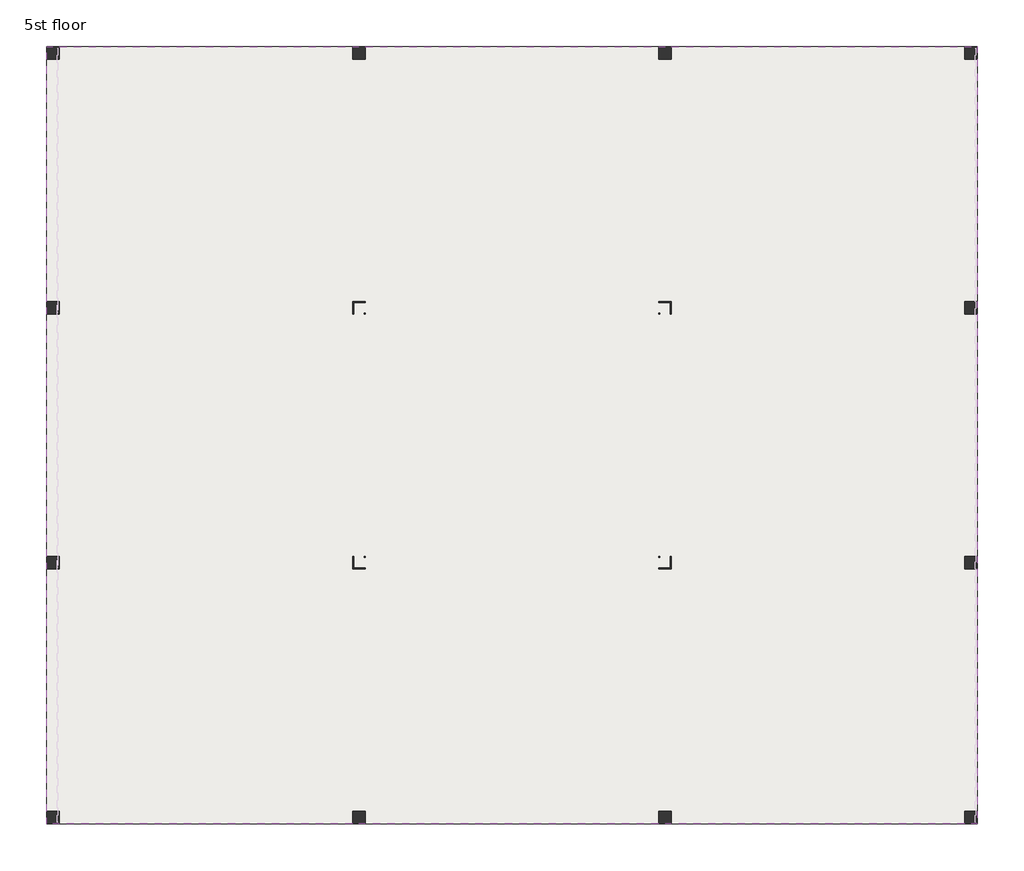
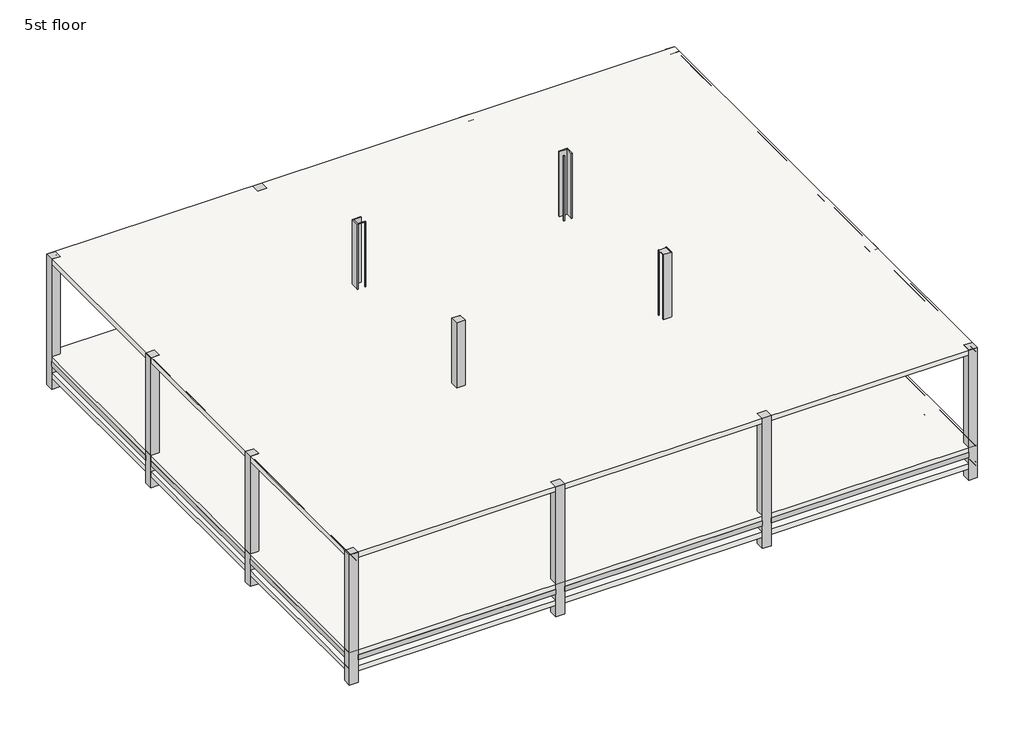
# One storey, part 1 of 2: 24 beams, 16 columns, 3 slabs.
"""IFC4 building model written with IfcOpenShell, lengths in millimetres."""

from ifc_helpers import new_model, si_unit, frame, origin, place, context, project, spatial, polyline, outline, extrude, faceted_brep, element, save

model = new_model("IFC4")

# Units and contexts
model_context = context("Model", 3, world=origin())
ifc_project = project(units=[si_unit("LENGTHUNIT", "METRE", prefix="MILLI")], contexts=[model_context])

# Site, building, storey
site = spatial("IfcSite", under=ifc_project)
building = spatial("IfcBuilding", under=site)
storey = spatial("IfcBuildingStorey", under=building, Name="5st floor", Elevation=19000.0)

# Beams
placement = place(None, origin())
element("IfcBeam", 1, ObjectType="Concrete-Rectangular Beam : 250 x 300mm", at=placement, inside=storey, context=model_context, shape_type="SweptSolid", body=[
    extrude(outline(polyline([(-8833.7181639, -5693.2383613), (-8833.7181639, -5443.2383613), (-3083.7181639, -5443.2383613), (-3083.7181639, -5693.2383613), (-8833.7181639, -5693.2383613)])), frame((0.0, 0.0, 18700.0), z_axis=(0.0, 0.0, 1.0), x_axis=(1.0, 0.0, 0.0)), (0.0, 0.0, 1.0), 150.0),
])
element("IfcBeam", 2, ObjectType="Concrete-Rectangular Beam : 250 x 300mm", at=placement, inside=storey, context=model_context, shape_type="SweptSolid", body=[
    extrude(outline(polyline([(-2833.7181639, -5693.2383613), (-2833.7181639, -5443.2383613), (2916.2818361, -5443.2383613), (2916.2818361, -5693.2383613), (-2833.7181639, -5693.2383613)])), frame((0.0, 0.0, 18700.0), z_axis=(0.0, 0.0, 1.0), x_axis=(1.0, 0.0, 0.0)), (0.0, 0.0, 1.0), 150.0),
])
element("IfcBeam", 3, ObjectType="Concrete-Rectangular Beam : 250 x 300mm", at=placement, inside=storey, context=model_context, shape_type="SweptSolid", body=[
    extrude(outline(polyline([(3166.2818361, -5693.2383613), (3166.2818361, -5443.2383613), (8916.2818361, -5443.2383613), (8916.2818361, -5693.2383613), (3166.2818361, -5693.2383613)])), frame((0.0, 0.0, 18700.0), z_axis=(0.0, 0.0, 1.0), x_axis=(1.0, 0.0, 0.0)), (0.0, 0.0, 1.0), 150.0),
])
element("IfcBeam", 4, ObjectType="Concrete-Rectangular Beam : 250 x 300mm", at=placement, inside=storey, context=model_context, shape_type="SweptSolid", body=[
    extrude(outline(polyline([(-8833.7181639, -10443.2383613), (-9083.7181639, -10443.2383613), (-9083.7181639, -5693.2383613), (-8833.7181639, -5693.2383613), (-8833.7181639, -10443.2383613)])), frame((0.0, 0.0, 18700.0), z_axis=(0.0, 0.0, 1.0), x_axis=(1.0, 0.0, 0.0)), (0.0, 0.0, 1.0), 150.0),
])
element("IfcBeam", 5, ObjectType="Concrete-Rectangular Beam : 250 x 300mm", at=placement, inside=storey, context=model_context, shape_type="SweptSolid", body=[
    extrude(outline(polyline([(-8833.7181639, -15443.2383613), (-9083.7181639, -15443.2383613), (-9083.7181639, -10693.2383613), (-8833.7181639, -10693.2383613), (-8833.7181639, -15443.2383613)])), frame((0.0, 0.0, 18700.0), z_axis=(0.0, 0.0, 1.0), x_axis=(1.0, 0.0, 0.0)), (0.0, 0.0, 1.0), 150.0),
])
element("IfcBeam", 6, ObjectType="Concrete-Rectangular Beam : 250 x 300mm", at=placement, inside=storey, context=model_context, shape_type="SweptSolid", body=[
    extrude(outline(polyline([(-8833.7181639, -20443.2383613), (-9083.7181639, -20443.2383613), (-9083.7181639, -15693.2383613), (-8833.7181639, -15693.2383613), (-8833.7181639, -20443.2383613)])), frame((0.0, 0.0, 18700.0), z_axis=(0.0, 0.0, 1.0), x_axis=(1.0, 0.0, 0.0)), (0.0, 0.0, 1.0), 150.0),
])
element("IfcBeam", 7, ObjectType="Concrete-Rectangular Beam : 250 x 300mm", at=placement, inside=storey, context=model_context, shape_type="SweptSolid", body=[
    extrude(outline(polyline([(-2833.7181639, -10443.2383613), (-3083.7181639, -10443.2383613), (-3083.7181639, -5693.2383613), (-2833.7181639, -5693.2383613), (-2833.7181639, -10443.2383613)])), frame((0.0, 0.0, 18700.0), z_axis=(0.0, 0.0, 1.0), x_axis=(1.0, 0.0, 0.0)), (0.0, 0.0, 1.0), 150.0),
])
element("IfcBeam", 8, ObjectType="Concrete-Rectangular Beam : 250 x 300mm", at=placement, inside=storey, context=model_context, shape_type="SweptSolid", body=[
    extrude(outline(polyline([(-3083.7181639, -15443.2383613), (-3083.7181639, -10693.2383613), (-3058.7181639, -10693.2383613), (-3058.7181639, -15443.2383613), (-3083.7181639, -15443.2383613)])), frame((0.0, 0.0, 18700.0), z_axis=(0.0, 0.0, 1.0), x_axis=(1.0, 0.0, 0.0)), (0.0, 0.0, 1.0), 150.0),
    extrude(outline(polyline([(-2833.7181639, -10693.2383613), (-2833.7181639, -15443.2383613), (-2858.7181639, -15443.2383613), (-2858.7181639, -10693.2383613), (-2833.7181639, -10693.2383613)])), frame((0.0, 0.0, 18700.0), z_axis=(0.0, 0.0, 1.0), x_axis=(1.0, 0.0, 0.0)), (0.0, 0.0, 1.0), 150.0),
])
element("IfcBeam", 9, ObjectType="Concrete-Rectangular Beam : 250 x 300mm", at=placement, inside=storey, context=model_context, shape_type="SweptSolid", body=[
    extrude(outline(polyline([(-2833.7181639, -20443.2383613), (-3083.7181639, -20443.2383613), (-3083.7181639, -15693.2383613), (-2833.7181639, -15693.2383613), (-2833.7181639, -20443.2383613)])), frame((0.0, 0.0, 18700.0), z_axis=(0.0, 0.0, 1.0), x_axis=(1.0, 0.0, 0.0)), (0.0, 0.0, 1.0), 150.0),
])
element("IfcBeam", 10, ObjectType="Concrete-Rectangular Beam : 250 x 300mm", at=placement, inside=storey, context=model_context, shape_type="SweptSolid", body=[
    extrude(outline(polyline([(3166.2818361, -10443.2383613), (2916.2818361, -10443.2383613), (2916.2818361, -5693.2383613), (3166.2818361, -5693.2383613), (3166.2818361, -10443.2383613)])), frame((0.0, 0.0, 18700.0), z_axis=(0.0, 0.0, 1.0), x_axis=(1.0, 0.0, 0.0)), (0.0, 0.0, 1.0), 150.0),
])
element("IfcBeam", 11, ObjectType="Concrete-Rectangular Beam : 250 x 300mm", at=placement, inside=storey, context=model_context, shape_type="SweptSolid", body=[
    extrude(outline(polyline([(2916.2818361, -15443.2383613), (2916.2818361, -10693.2383613), (2941.2818361, -10693.2383613), (2941.2818361, -15443.2383613), (2916.2818361, -15443.2383613)])), frame((0.0, 0.0, 18700.0), z_axis=(0.0, 0.0, 1.0), x_axis=(1.0, 0.0, 0.0)), (0.0, 0.0, 1.0), 150.0),
    extrude(outline(polyline([(3166.2818361, -10693.2383613), (3166.2818361, -15443.2383613), (3141.2818361, -15443.2383613), (3141.2818361, -10693.2383613), (3166.2818361, -10693.2383613)])), frame((0.0, 0.0, 18700.0), z_axis=(0.0, 0.0, 1.0), x_axis=(1.0, 0.0, 0.0)), (0.0, 0.0, 1.0), 150.0),
])
element("IfcBeam", 12, ObjectType="Concrete-Rectangular Beam : 250 x 300mm", at=placement, inside=storey, context=model_context, shape_type="SweptSolid", body=[
    extrude(outline(polyline([(3166.2818361, -20443.2383613), (2916.2818361, -20443.2383613), (2916.2818361, -15693.2383613), (3166.2818361, -15693.2383613), (3166.2818361, -20443.2383613)])), frame((0.0, 0.0, 18700.0), z_axis=(0.0, 0.0, 1.0), x_axis=(1.0, 0.0, 0.0)), (0.0, 0.0, 1.0), 150.0),
])
element("IfcBeam", 13, ObjectType="Concrete-Rectangular Beam : 250 x 300mm", at=placement, inside=storey, context=model_context, shape_type="SweptSolid", body=[
    extrude(outline(polyline([(9166.2818361, -10443.2383613), (8916.2818361, -10443.2383613), (8916.2818361, -5693.2383613), (9166.2818361, -5693.2383613), (9166.2818361, -10443.2383613)])), frame((0.0, 0.0, 18700.0), z_axis=(0.0, 0.0, 1.0), x_axis=(1.0, 0.0, 0.0)), (0.0, 0.0, 1.0), 150.0),
])
element("IfcBeam", 14, ObjectType="Concrete-Rectangular Beam : 250 x 300mm", at=placement, inside=storey, context=model_context, shape_type="SweptSolid", body=[
    extrude(outline(polyline([(9166.2818361, -15443.2383613), (8916.2818361, -15443.2383613), (8916.2818361, -10693.2383613), (9166.2818361, -10693.2383613), (9166.2818361, -15443.2383613)])), frame((0.0, 0.0, 18700.0), z_axis=(0.0, 0.0, 1.0), x_axis=(1.0, 0.0, 0.0)), (0.0, 0.0, 1.0), 150.0),
])
element("IfcBeam", 15, ObjectType="Concrete-Rectangular Beam : 250 x 300mm", at=placement, inside=storey, context=model_context, shape_type="SweptSolid", body=[
    extrude(outline(polyline([(9166.2818361, -20443.2383613), (8916.2818361, -20443.2383613), (8916.2818361, -15693.2383613), (9166.2818361, -15693.2383613), (9166.2818361, -20443.2383613)])), frame((0.0, 0.0, 18700.0), z_axis=(0.0, 0.0, 1.0), x_axis=(1.0, 0.0, 0.0)), (0.0, 0.0, 1.0), 150.0),
])
element("IfcBeam", 16, ObjectType="Concrete-Rectangular Beam : 250 x 300mm", at=placement, inside=storey, context=model_context, shape_type="SweptSolid", body=[
    extrude(outline(polyline([(-8833.7181639, -20693.2383613), (-8833.7181639, -20443.2383613), (-3083.7181639, -20443.2383613), (-3083.7181639, -20693.2383613), (-8833.7181639, -20693.2383613)])), frame((0.0, 0.0, 18700.0), z_axis=(0.0, 0.0, 1.0), x_axis=(1.0, 0.0, 0.0)), (0.0, 0.0, 1.0), 150.0),
])
element("IfcBeam", 17, ObjectType="Concrete-Rectangular Beam : 250 x 300mm", at=placement, inside=storey, context=model_context, shape_type="SweptSolid", body=[
    extrude(outline(polyline([(-2833.7181639, -20693.2383613), (-2833.7181639, -20443.2383613), (2916.2818361, -20443.2383613), (2916.2818361, -20693.2383613), (-2833.7181639, -20693.2383613)])), frame((0.0, 0.0, 18700.0), z_axis=(0.0, 0.0, 1.0), x_axis=(1.0, 0.0, 0.0)), (0.0, 0.0, 1.0), 150.0),
])
element("IfcBeam", 18, ObjectType="Concrete-Rectangular Beam : 250 x 300mm", at=placement, inside=storey, context=model_context, shape_type="SweptSolid", body=[
    extrude(outline(polyline([(3166.2818361, -20693.2383613), (3166.2818361, -20443.2383613), (8916.2818361, -20443.2383613), (8916.2818361, -20693.2383613), (3166.2818361, -20693.2383613)])), frame((0.0, 0.0, 18700.0), z_axis=(0.0, 0.0, 1.0), x_axis=(1.0, 0.0, 0.0)), (0.0, 0.0, 1.0), 150.0),
])
element("IfcBeam", 19, ObjectType="Concrete-Rectangular Beam : 250 x 300mm", at=placement, inside=storey, context=model_context, shape_type="SweptSolid", body=[
    extrude(outline(polyline([(-8833.7181639, -15693.2383613), (-8833.7181639, -15443.2383613), (-3083.7181639, -15443.2383613), (-3083.7181639, -15693.2383613), (-8833.7181639, -15693.2383613)])), frame((0.0, 0.0, 18700.0), z_axis=(0.0, 0.0, 1.0), x_axis=(1.0, 0.0, 0.0)), (0.0, 0.0, 1.0), 150.0),
])
element("IfcBeam", 20, ObjectType="Concrete-Rectangular Beam : 250 x 300mm", at=placement, inside=storey, context=model_context, shape_type="SweptSolid", body=[
    extrude(outline(polyline([(2916.2818361, -15693.2383613), (-2833.7181639, -15693.2383613), (-2833.7181639, -15668.2383613), (2916.2818361, -15668.2383613), (2916.2818361, -15693.2383613)])), frame((0.0, 0.0, 18700.0), z_axis=(0.0, 0.0, 1.0), x_axis=(1.0, 0.0, 0.0)), (0.0, 0.0, 1.0), 150.0),
    extrude(outline(polyline([(-2833.7181639, -15443.2383613), (2916.2818361, -15443.2383613), (2916.2818361, -15468.2383613), (-2833.7181639, -15468.2383613), (-2833.7181639, -15443.2383613)])), frame((0.0, 0.0, 18700.0), z_axis=(0.0, 0.0, 1.0), x_axis=(1.0, 0.0, 0.0)), (0.0, 0.0, 1.0), 150.0),
])
element("IfcBeam", 21, ObjectType="Concrete-Rectangular Beam : 250 x 300mm", at=placement, inside=storey, context=model_context, shape_type="SweptSolid", body=[
    extrude(outline(polyline([(3166.2818361, -15693.2383613), (3166.2818361, -15443.2383613), (8916.2818361, -15443.2383613), (8916.2818361, -15693.2383613), (3166.2818361, -15693.2383613)])), frame((0.0, 0.0, 18700.0), z_axis=(0.0, 0.0, 1.0), x_axis=(1.0, 0.0, 0.0)), (0.0, 0.0, 1.0), 150.0),
])
element("IfcBeam", 22, ObjectType="Concrete-Rectangular Beam : 250 x 300mm", at=placement, inside=storey, context=model_context, shape_type="SweptSolid", body=[
    extrude(outline(polyline([(-8833.7181639, -10693.2383613), (-8833.7181639, -10443.2383613), (-3083.7181639, -10443.2383613), (-3083.7181639, -10693.2383613), (-8833.7181639, -10693.2383613)])), frame((0.0, 0.0, 18700.0), z_axis=(0.0, 0.0, 1.0), x_axis=(1.0, 0.0, 0.0)), (0.0, 0.0, 1.0), 150.0),
])
element("IfcBeam", 23, ObjectType="Concrete-Rectangular Beam : 250 x 300mm", at=placement, inside=storey, context=model_context, shape_type="SweptSolid", body=[
    extrude(outline(polyline([(2916.2818361, -10693.2383613), (-2833.7181639, -10693.2383613), (-2833.7181639, -10668.2383613), (2916.2818361, -10668.2383613), (2916.2818361, -10693.2383613)])), frame((0.0, 0.0, 18700.0), z_axis=(0.0, 0.0, 1.0), x_axis=(1.0, 0.0, 0.0)), (0.0, 0.0, 1.0), 150.0),
    extrude(outline(polyline([(-2833.7181639, -10443.2383613), (2916.2818361, -10443.2383613), (2916.2818361, -10468.2383613), (-2833.7181639, -10468.2383613), (-2833.7181639, -10443.2383613)])), frame((0.0, 0.0, 18700.0), z_axis=(0.0, 0.0, 1.0), x_axis=(1.0, 0.0, 0.0)), (0.0, 0.0, 1.0), 150.0),
])
element("IfcBeam", 24, ObjectType="Concrete-Rectangular Beam : 250 x 300mm", at=placement, inside=storey, context=model_context, shape_type="SweptSolid", body=[
    extrude(outline(polyline([(3166.2818361, -10693.2383613), (3166.2818361, -10443.2383613), (8916.2818361, -10443.2383613), (8916.2818361, -10693.2383613), (3166.2818361, -10693.2383613)])), frame((0.0, 0.0, 18700.0), z_axis=(0.0, 0.0, 1.0), x_axis=(1.0, 0.0, 0.0)), (0.0, 0.0, 1.0), 150.0),
])

# Columns
element("IfcColumn", 25, ObjectType="Concrete-Rectangular-Column : 250x250 mm", at=placement, inside=storey, context=model_context, shape_type="Brep", body=[
    faceted_brep([(-8833.7181639, -20443.2383613, 22000.0), (-9083.7181639, -20443.2383613, 22000.0), (-9083.7181639, -20693.2383613, 22000.0), (-8833.7181639, -20693.2383613, 22000.0), (-8833.7181639, -20443.2383613, 18000.0), (-8833.7181639, -20693.2383613, 18000.0), (-9083.7181639, -20693.2383613, 18000.0), (-9083.7181639, -20443.2383613, 18000.0), (-8833.7181639, -20443.2383613, 18350.0), (-8833.7181639, -20443.2383613, 18200.0), (-9083.7181639, -20443.2383613, 18200.0), (-9083.7181639, -20443.2383613, 18350.0), (-8833.7181639, -20693.2383613, 18200.0), (-8833.7181639, -20693.2383613, 18350.0)], [[[0, 1, 2, 3]], [[4, 5, 6, 7]], [[1, 0, 8, 9, 4, 7, 10, 11]], [[2, 1, 11, 10, 7, 6]], [[3, 2, 6, 5, 12, 13]], [[0, 3, 13, 12, 5, 4, 9, 8]]]),
])
element("IfcColumn", 26, ObjectType="Concrete-Rectangular-Column : 250x250 mm", at=placement, inside=storey, context=model_context, shape_type="Brep", body=[
    faceted_brep([(-8833.7181639, -15443.2383613, 22000.0), (-9083.7181639, -15443.2383613, 22000.0), (-9083.7181639, -15693.2383613, 22000.0), (-8833.7181639, -15693.2383613, 22000.0), (-8833.7181639, -15443.2383613, 18000.0), (-8833.7181639, -15693.2383613, 18000.0), (-9083.7181639, -15693.2383613, 18000.0), (-9083.7181639, -15443.2383613, 18000.0), (-8833.7181639, -15443.2383613, 18350.0), (-8833.7181639, -15443.2383613, 18200.0), (-9083.7181639, -15443.2383613, 18200.0), (-9083.7181639, -15443.2383613, 18350.0), (-9083.7181639, -15693.2383613, 18200.0), (-9083.7181639, -15693.2383613, 18350.0), (-8833.7181639, -15693.2383613, 18200.0), (-8833.7181639, -15693.2383613, 18350.0)], [[[0, 1, 2, 3]], [[4, 5, 6, 7]], [[1, 0, 8, 9, 4, 7, 10, 11]], [[2, 1, 11, 10, 7, 6, 12, 13]], [[3, 2, 13, 12, 6, 5, 14, 15]], [[0, 3, 15, 14, 5, 4, 9, 8]]]),
])
element("IfcColumn", 27, ObjectType="Concrete-Rectangular-Column : 250x250 mm", at=placement, inside=storey, context=model_context, shape_type="Brep", body=[
    faceted_brep([(-8833.7181639, -10443.2383613, 22000.0), (-9083.7181639, -10443.2383613, 22000.0), (-9083.7181639, -10693.2383613, 22000.0), (-8833.7181639, -10693.2383613, 22000.0), (-8833.7181639, -10443.2383613, 18000.0), (-8833.7181639, -10693.2383613, 18000.0), (-9083.7181639, -10693.2383613, 18000.0), (-9083.7181639, -10443.2383613, 18000.0), (-8833.7181639, -10443.2383613, 18350.0), (-8833.7181639, -10443.2383613, 18200.0), (-9083.7181639, -10443.2383613, 18200.0), (-9083.7181639, -10443.2383613, 18350.0), (-9083.7181639, -10693.2383613, 18200.0), (-9083.7181639, -10693.2383613, 18350.0), (-8833.7181639, -10693.2383613, 18200.0), (-8833.7181639, -10693.2383613, 18350.0)], [[[0, 1, 2, 3]], [[4, 5, 6, 7]], [[1, 0, 8, 9, 4, 7, 10, 11]], [[2, 1, 11, 10, 7, 6, 12, 13]], [[3, 2, 13, 12, 6, 5, 14, 15]], [[0, 3, 15, 14, 5, 4, 9, 8]]]),
])
element("IfcColumn", 28, ObjectType="Concrete-Rectangular-Column : 250x250 mm", at=placement, inside=storey, context=model_context, shape_type="Brep", body=[
    faceted_brep([(-8833.7181639, -5443.2383613, 22000.0), (-9083.7181639, -5443.2383613, 22000.0), (-9083.7181639, -5693.2383613, 22000.0), (-8833.7181639, -5693.2383613, 22000.0), (-8833.7181639, -5443.2383613, 18000.0), (-8833.7181639, -5693.2383613, 18000.0), (-9083.7181639, -5693.2383613, 18000.0), (-9083.7181639, -5443.2383613, 18000.0), (-8833.7181639, -5443.2383613, 18350.0), (-8833.7181639, -5443.2383613, 18200.0), (-9083.7181639, -5693.2383613, 18200.0), (-9083.7181639, -5693.2383613, 18350.0), (-8833.7181639, -5693.2383613, 18200.0), (-8833.7181639, -5693.2383613, 18350.0)], [[[0, 1, 2, 3]], [[4, 5, 6, 7]], [[1, 0, 8, 9, 4, 7]], [[2, 1, 7, 6, 10, 11]], [[3, 2, 11, 10, 6, 5, 12, 13]], [[0, 3, 13, 12, 5, 4, 9, 8]]]),
])
element("IfcColumn", 29, ObjectType="Concrete-Rectangular-Column : 250x250 mm", at=placement, inside=storey, context=model_context, shape_type="Brep", body=[
    faceted_brep([(-2833.7181639, -20443.2383613, 22000.0), (-3083.7181639, -20443.2383613, 22000.0), (-3083.7181639, -20693.2383613, 22000.0), (-2833.7181639, -20693.2383613, 22000.0), (-2833.7181639, -20443.2383613, 18000.0), (-2833.7181639, -20693.2383613, 18000.0), (-3083.7181639, -20693.2383613, 18000.0), (-3083.7181639, -20443.2383613, 18000.0), (-2833.7181639, -20443.2383613, 18350.0), (-2833.7181639, -20443.2383613, 18200.0), (-3083.7181639, -20443.2383613, 18200.0), (-3083.7181639, -20443.2383613, 18350.0), (-3083.7181639, -20693.2383613, 18200.0), (-3083.7181639, -20693.2383613, 18350.0), (-2833.7181639, -20693.2383613, 18200.0), (-2833.7181639, -20693.2383613, 18350.0)], [[[0, 1, 2, 3]], [[4, 5, 6, 7]], [[1, 0, 8, 9, 4, 7, 10, 11]], [[2, 1, 11, 10, 7, 6, 12, 13]], [[3, 2, 13, 12, 6, 5, 14, 15]], [[0, 3, 15, 14, 5, 4, 9, 8]]]),
])
element("IfcColumn", 30, ObjectType="Concrete-Rectangular-Column : 250x250 mm", at=placement, inside=storey, context=model_context, shape_type="Brep", body=[
    faceted_brep([(-2833.7181639, -15443.2383613, 24000.0), (-3083.7181639, -15443.2383613, 24000.0), (-3083.7181639, -15693.2383613, 24000.0), (-2833.7181639, -15693.2383613, 24000.0), (-2833.7181639, -15443.2383613, 18000.0), (-2833.7181639, -15468.2383613, 18000.0), (-2858.7181639, -15468.2383613, 18000.0), (-2858.7181639, -15443.2383613, 18000.0), (-2833.7181639, -15443.2383613, 18350.0), (-2833.7181639, -15443.2383613, 18200.0), (-2858.7181639, -15443.2383613, 18200.0), (-2858.7181639, -15443.2383613, 18350.0), (-2858.7181639, -15443.2383613, 23998.7852478), (-3058.7181639, -15443.2383613, 23998.7852478), (-3058.7181639, -15443.2383613, 18350.0), (-3058.7181639, -15443.2383613, 18200.0), (-3058.7181639, -15443.2383613, 18000.0), (-3083.7181639, -15443.2383613, 18000.0), (-3083.7181639, -15443.2383613, 18200.0), (-3083.7181639, -15443.2383613, 18350.0), (-3083.7181639, -15693.2383613, 18000.0), (-3083.7181639, -15693.2383613, 18200.0), (-3083.7181639, -15693.2383613, 18350.0), (-2833.7181639, -15693.2383613, 18000.0), (-2833.7181639, -15693.2383613, 18200.0), (-2833.7181639, -15693.2383613, 18350.0), (-2833.7181639, -15668.2383613, 18000.0), (-2833.7181639, -15668.2383613, 18200.0), (-2833.7181639, -15668.2383613, 18350.0), (-2833.7181639, -15668.2383613, 23998.7852478), (-2833.7181639, -15468.2383613, 23998.7852478), (-2833.7181639, -15468.2383613, 18350.0), (-2833.7181639, -15468.2383613, 18200.0), (-2858.7181639, -15468.2383613, 23998.7852478), (-3058.7181639, -15668.2383613, 18000.0), (-3058.7181639, -15668.2383613, 23998.7852478), (-3058.7181639, -15468.2383613, 23998.7852478)], [[[0, 1, 2, 3]], [[4, 5, 6, 7]], [[1, 0, 8, 9, 4, 7, 10, 11, 12, 13, 14, 15, 16, 17, 18, 19]], [[2, 1, 19, 18, 17, 20, 21, 22]], [[3, 2, 22, 21, 20, 23, 24, 25]], [[0, 3, 25, 24, 23, 26, 27, 28, 29, 30, 31, 32, 5, 4, 9, 8]], [[5, 32, 31, 30, 33, 6]], [[34, 35, 29, 28, 27, 26]], [[35, 34, 16, 15, 14, 13, 36]], [[33, 12, 11, 10, 7, 6]], [[23, 20, 17, 16, 34, 26]], [[35, 36, 13, 12, 33, 30, 29]]]),
])
element("IfcColumn", 31, ObjectType="Concrete-Rectangular-Column : 250x250 mm", at=placement, inside=storey, context=model_context, shape_type="Brep", body=[
    faceted_brep([(-2833.7181639, -10443.2383613, 24000.0), (-3083.7181639, -10443.2383613, 24000.0), (-3083.7181639, -10693.2383613, 24000.0), (-2833.7181639, -10693.2383613, 24000.0), (-2833.7181639, -10668.2383613, 24000.0), (-3058.7181639, -10668.2383613, 24000.0), (-3058.7181639, -10468.2383613, 24000.0), (-2833.7181639, -10468.2383613, 24000.0), (-3083.7181639, -10693.2383613, 18000.0), (-3083.7181639, -10443.2383613, 18000.0), (-2833.7181639, -10443.2383613, 18000.0), (-2833.7181639, -10468.2383613, 18000.0), (-3058.7181639, -10468.2383613, 18000.0), (-3058.7181639, -10693.2383613, 18000.0), (-2833.7181639, -10443.2383613, 18350.0), (-2833.7181639, -10443.2383613, 18200.0), (-3083.7181639, -10443.2383613, 18200.0), (-3083.7181639, -10443.2383613, 18350.0), (-3083.7181639, -10693.2383613, 18200.0), (-3083.7181639, -10693.2383613, 18350.0), (-3058.7181639, -10693.2383613, 18200.0), (-3058.7181639, -10693.2383613, 18350.0), (-3058.7181639, -10693.2383613, 23998.7852478), (-2858.7181639, -10693.2383613, 23998.7852478), (-2858.7181639, -10693.2383613, 18350.0), (-2858.7181639, -10693.2383613, 18200.0), (-2858.7181639, -10693.2383613, 18000.0), (-2833.7181639, -10693.2383613, 18000.0), (-2833.7181639, -10693.2383613, 18200.0), (-2833.7181639, -10693.2383613, 18350.0), (-2833.7181639, -10468.2383613, 18350.0), (-2833.7181639, -10468.2383613, 18200.0), (-2833.7181639, -10668.2383613, 18350.0), (-2833.7181639, -10668.2383613, 18200.0), (-2833.7181639, -10668.2383613, 18000.0), (-2858.7181639, -10668.2383613, 18000.0), (-2858.7181639, -10668.2383613, 23998.7852478), (-3058.7181639, -10668.2383613, 23998.7852478)], [[[0, 1, 2, 3, 4, 5, 6, 7]], [[8, 9, 10, 11, 12, 13]], [[1, 0, 14, 15, 10, 9, 16, 17]], [[2, 1, 17, 16, 9, 8, 18, 19]], [[3, 2, 19, 18, 8, 13, 20, 21, 22, 23, 24, 25, 26, 27, 28, 29]], [[10, 15, 14, 0, 7, 30, 31, 11]], [[4, 32, 33, 34, 35, 36, 37, 5]], [[12, 11, 31, 30, 7, 6]], [[12, 6, 5, 37, 22, 21, 20, 13]], [[23, 36, 35, 26, 25, 24]], [[34, 27, 26, 35]], [[3, 29, 28, 27, 34, 33, 32, 4]], [[22, 37, 36, 23]]]),
])
element("IfcColumn", 32, ObjectType="Concrete-Rectangular-Column : 250x250 mm", at=placement, inside=storey, context=model_context, shape_type="Brep", body=[
    faceted_brep([(-2833.7181639, -5443.2383613, 22000.0), (-3083.7181639, -5443.2383613, 22000.0), (-3083.7181639, -5693.2383613, 22000.0), (-2833.7181639, -5693.2383613, 22000.0), (-2833.7181639, -5443.2383613, 18000.0), (-2833.7181639, -5693.2383613, 18000.0), (-3083.7181639, -5693.2383613, 18000.0), (-3083.7181639, -5443.2383613, 18000.0), (-2833.7181639, -5443.2383613, 18350.0), (-2833.7181639, -5443.2383613, 18200.0), (-3083.7181639, -5443.2383613, 18200.0), (-3083.7181639, -5443.2383613, 18350.0), (-3083.7181639, -5693.2383613, 18200.0), (-3083.7181639, -5693.2383613, 18350.0), (-2833.7181639, -5693.2383613, 18200.0), (-2833.7181639, -5693.2383613, 18350.0)], [[[0, 1, 2, 3]], [[4, 5, 6, 7]], [[1, 0, 8, 9, 4, 7, 10, 11]], [[2, 1, 11, 10, 7, 6, 12, 13]], [[3, 2, 13, 12, 6, 5, 14, 15]], [[0, 3, 15, 14, 5, 4, 9, 8]]]),
])
element("IfcColumn", 33, ObjectType="Concrete-Rectangular-Column : 250x250 mm", at=placement, inside=storey, context=model_context, shape_type="Brep", body=[
    faceted_brep([(3166.2818361, -20443.2383613, 22000.0), (2916.2818361, -20443.2383613, 22000.0), (2916.2818361, -20693.2383613, 22000.0), (3166.2818361, -20693.2383613, 22000.0), (3166.2818361, -20443.2383613, 18000.0), (3166.2818361, -20693.2383613, 18000.0), (2916.2818361, -20693.2383613, 18000.0), (2916.2818361, -20443.2383613, 18000.0), (3166.2818361, -20443.2383613, 18350.0), (3166.2818361, -20443.2383613, 18200.0), (2916.2818361, -20443.2383613, 18200.0), (2916.2818361, -20443.2383613, 18350.0), (2916.2818361, -20693.2383613, 18200.0), (2916.2818361, -20693.2383613, 18350.0), (3166.2818361, -20693.2383613, 18200.0), (3166.2818361, -20693.2383613, 18350.0)], [[[0, 1, 2, 3]], [[4, 5, 6, 7]], [[1, 0, 8, 9, 4, 7, 10, 11]], [[2, 1, 11, 10, 7, 6, 12, 13]], [[3, 2, 13, 12, 6, 5, 14, 15]], [[0, 3, 15, 14, 5, 4, 9, 8]]]),
])
element("IfcColumn", 34, ObjectType="Concrete-Rectangular-Column : 250x250 mm", at=placement, inside=storey, context=model_context, shape_type="Brep", body=[
    faceted_brep([(2916.2818361, -15443.2383613, 24000.0), (2916.2818361, -15693.2383613, 24000.0), (3166.2818361, -15693.2383613, 24000.0), (3166.2818361, -15443.2383613, 24000.0), (3141.2818361, -15443.2383613, 24000.0), (3141.2818361, -15468.2383613, 24000.0), (2941.2818361, -15468.2383613, 24000.0), (2941.2818361, -15443.2383613, 24000.0), (2916.2818361, -15468.2383613, 18000.0), (2916.2818361, -15443.2383613, 18000.0), (2941.2818361, -15443.2383613, 18000.0), (2941.2818361, -15468.2383613, 18000.0), (3166.2818361, -15443.2383613, 18350.0), (3166.2818361, -15443.2383613, 18200.0), (3166.2818361, -15443.2383613, 18000.0), (3141.2818361, -15443.2383613, 18000.0), (3141.2818361, -15443.2383613, 18200.0), (3141.2818361, -15443.2383613, 18350.0), (2916.2818361, -15443.2383613, 18350.0), (2916.2818361, -15443.2383613, 18200.0), (2916.2818361, -15468.2383613, 18200.0), (2916.2818361, -15468.2383613, 18350.0), (2916.2818361, -15468.2383613, 23998.7852478), (2916.2818361, -15668.2383613, 23998.7852478), (2916.2818361, -15668.2383613, 18350.0), (2916.2818361, -15668.2383613, 18200.0), (2916.2818361, -15668.2383613, 18000.0), (2916.2818361, -15693.2383613, 18000.0), (2916.2818361, -15693.2383613, 18200.0), (2916.2818361, -15693.2383613, 18350.0), (3166.2818361, -15693.2383613, 18000.0), (3166.2818361, -15693.2383613, 18200.0), (3166.2818361, -15693.2383613, 18350.0), (2941.2818361, -15468.2383613, 23998.7852478), (3141.2818361, -15668.2383613, 23998.7852478), (3141.2818361, -15668.2383613, 18000.0), (3141.2818361, -15468.2383613, 23998.7852478), (2941.2818361, -15443.2383613, 18200.0), (2941.2818361, -15443.2383613, 18350.0)], [[[0, 1, 2, 3, 4, 5, 6, 7]], [[8, 9, 10, 11]], [[3, 12, 13, 14, 15, 16, 17, 4]], [[1, 0, 18, 19, 9, 8, 20, 21, 22, 23, 24, 25, 26, 27, 28, 29]], [[2, 1, 29, 28, 27, 30, 31, 32]], [[3, 2, 32, 31, 30, 14, 13, 12]], [[22, 21, 20, 8, 11, 33]], [[34, 35, 26, 25, 24, 23]], [[34, 36, 5, 4, 17, 16, 15, 35]], [[6, 33, 11, 10, 37, 38, 7]], [[5, 36, 33, 6]], [[14, 30, 27, 26, 35, 15]], [[9, 19, 18, 0, 7, 38, 37, 10]], [[36, 34, 23, 22, 33]]]),
])
element("IfcColumn", 35, ObjectType="Concrete-Rectangular-Column : 250x250 mm", at=placement, inside=storey, context=model_context, shape_type="Brep", body=[
    faceted_brep([(3166.2818361, -10443.2383613, 24000.0), (2916.2818361, -10443.2383613, 24000.0), (2916.2818361, -10468.2383613, 24000.0), (3141.2818361, -10468.2383613, 24000.0), (3141.2818361, -10693.2383613, 24000.0), (3166.2818361, -10693.2383613, 24000.0), (3166.2818361, -10443.2383613, 18350.0), (3166.2818361, -10443.2383613, 18200.0), (3166.2818361, -10443.2383613, 18000.0), (2916.2818361, -10443.2383613, 18000.0), (2916.2818361, -10443.2383613, 18200.0), (2916.2818361, -10443.2383613, 18350.0), (2916.2818361, -10468.2383613, 18000.0), (2916.2818361, -10468.2383613, 18200.0), (2916.2818361, -10468.2383613, 18350.0), (3166.2818361, -10693.2383613, 18350.0), (3166.2818361, -10693.2383613, 18200.0), (3166.2818361, -10693.2383613, 18000.0), (3141.2818361, -10468.2383613, 18000.0), (3141.2818361, -10693.2383613, 18000.0), (3141.2818361, -10693.2383613, 18200.0), (3141.2818361, -10693.2383613, 18350.0)], [[[0, 1, 2, 3, 4, 5]], [[1, 0, 6, 7, 8, 9, 10, 11]], [[1, 11, 10, 9, 12, 13, 14, 2]], [[0, 5, 15, 16, 17, 8, 7, 6]], [[12, 18, 3, 2, 14, 13]], [[19, 20, 21, 4, 3, 18]], [[8, 17, 19, 18, 12, 9]], [[17, 16, 15, 5, 4, 21, 20, 19]]]),
    faceted_brep([(2916.2818361, -10693.2383613, 18000.0), (2916.2818361, -10668.2383613, 18000.0), (2941.2818361, -10668.2383613, 18000.0), (2941.2818361, -10693.2383613, 18000.0), (2916.2818361, -10693.2383613, 24000.0), (2916.2818361, -10693.2383613, 18350.0), (2916.2818361, -10693.2383613, 18200.0), (2941.2818361, -10693.2383613, 18200.0), (2941.2818361, -10693.2383613, 18350.0), (2941.2818361, -10693.2383613, 24000.0), (2916.2818361, -10668.2383613, 18200.0), (2916.2818361, -10668.2383613, 18350.0), (2916.2818361, -10668.2383613, 24000.0), (2941.2818361, -10668.2383613, 24000.0)], [[[0, 1, 2, 3]], [[4, 5, 6, 0, 3, 7, 8, 9]], [[1, 10, 11, 12, 13, 2]], [[13, 9, 8, 7, 3, 2]], [[0, 6, 5, 4, 12, 11, 10, 1]], [[12, 4, 9, 13]]]),
])
element("IfcColumn", 36, ObjectType="Concrete-Rectangular-Column : 250x250 mm", at=placement, inside=storey, context=model_context, shape_type="Brep", body=[
    faceted_brep([(3166.2818361, -5443.2383613, 22000.0), (2916.2818361, -5443.2383613, 22000.0), (2916.2818361, -5693.2383613, 22000.0), (3166.2818361, -5693.2383613, 22000.0), (3166.2818361, -5443.2383613, 18000.0), (3166.2818361, -5693.2383613, 18000.0), (2916.2818361, -5693.2383613, 18000.0), (2916.2818361, -5443.2383613, 18000.0), (3166.2818361, -5443.2383613, 18350.0), (3166.2818361, -5443.2383613, 18200.0), (2916.2818361, -5443.2383613, 18200.0), (2916.2818361, -5443.2383613, 18350.0), (2916.2818361, -5693.2383613, 18200.0), (2916.2818361, -5693.2383613, 18350.0), (3166.2818361, -5693.2383613, 18200.0), (3166.2818361, -5693.2383613, 18350.0)], [[[0, 1, 2, 3]], [[4, 5, 6, 7]], [[1, 0, 8, 9, 4, 7, 10, 11]], [[2, 1, 11, 10, 7, 6, 12, 13]], [[3, 2, 13, 12, 6, 5, 14, 15]], [[0, 3, 15, 14, 5, 4, 9, 8]]]),
])
element("IfcColumn", 37, ObjectType="Concrete-Rectangular-Column : 250x250 mm", at=placement, inside=storey, context=model_context, shape_type="Brep", body=[
    faceted_brep([(9166.2818361, -20443.2383613, 22000.0), (8916.2818361, -20443.2383613, 22000.0), (8916.2818361, -20693.2383613, 22000.0), (9166.2818361, -20693.2383613, 22000.0), (9166.2818361, -20443.2383613, 18000.0), (9166.2818361, -20693.2383613, 18000.0), (8916.2818361, -20693.2383613, 18000.0), (8916.2818361, -20443.2383613, 18000.0), (9166.2818361, -20443.2383613, 18350.0), (9166.2818361, -20443.2383613, 18200.0), (8916.2818361, -20443.2383613, 18200.0), (8916.2818361, -20443.2383613, 18350.0), (8916.2818361, -20693.2383613, 18200.0), (8916.2818361, -20693.2383613, 18350.0)], [[[0, 1, 2, 3]], [[4, 5, 6, 7]], [[1, 0, 8, 9, 4, 7, 10, 11]], [[2, 1, 11, 10, 7, 6, 12, 13]], [[3, 2, 13, 12, 6, 5]], [[0, 3, 5, 4, 9, 8]]]),
])
element("IfcColumn", 38, ObjectType="Concrete-Rectangular-Column : 250x250 mm", at=placement, inside=storey, context=model_context, shape_type="Brep", body=[
    faceted_brep([(9166.2818361, -15443.2383613, 22000.0), (8916.2818361, -15443.2383613, 22000.0), (8916.2818361, -15693.2383613, 22000.0), (9166.2818361, -15693.2383613, 22000.0), (9166.2818361, -15443.2383613, 18000.0), (9166.2818361, -15693.2383613, 18000.0), (8916.2818361, -15693.2383613, 18000.0), (8916.2818361, -15443.2383613, 18000.0), (9166.2818361, -15443.2383613, 18350.0), (9166.2818361, -15443.2383613, 18200.0), (8916.2818361, -15443.2383613, 18200.0), (8916.2818361, -15443.2383613, 18350.0), (8916.2818361, -15693.2383613, 18200.0), (8916.2818361, -15693.2383613, 18350.0), (9166.2818361, -15693.2383613, 18200.0), (9166.2818361, -15693.2383613, 18350.0)], [[[0, 1, 2, 3]], [[4, 5, 6, 7]], [[1, 0, 8, 9, 4, 7, 10, 11]], [[2, 1, 11, 10, 7, 6, 12, 13]], [[3, 2, 13, 12, 6, 5, 14, 15]], [[0, 3, 15, 14, 5, 4, 9, 8]]]),
])
element("IfcColumn", 39, ObjectType="Concrete-Rectangular-Column : 250x250 mm", at=placement, inside=storey, context=model_context, shape_type="Brep", body=[
    faceted_brep([(9166.2818361, -10443.2383613, 22000.0), (8916.2818361, -10443.2383613, 22000.0), (8916.2818361, -10693.2383613, 22000.0), (9166.2818361, -10693.2383613, 22000.0), (9166.2818361, -10443.2383613, 18000.0), (9166.2818361, -10693.2383613, 18000.0), (8916.2818361, -10693.2383613, 18000.0), (8916.2818361, -10443.2383613, 18000.0), (9166.2818361, -10443.2383613, 18350.0), (9166.2818361, -10443.2383613, 18200.0), (8916.2818361, -10443.2383613, 18200.0), (8916.2818361, -10443.2383613, 18350.0), (8916.2818361, -10693.2383613, 18200.0), (8916.2818361, -10693.2383613, 18350.0), (9166.2818361, -10693.2383613, 18200.0), (9166.2818361, -10693.2383613, 18350.0)], [[[0, 1, 2, 3]], [[4, 5, 6, 7]], [[1, 0, 8, 9, 4, 7, 10, 11]], [[2, 1, 11, 10, 7, 6, 12, 13]], [[3, 2, 13, 12, 6, 5, 14, 15]], [[0, 3, 15, 14, 5, 4, 9, 8]]]),
])
element("IfcColumn", 40, ObjectType="Concrete-Rectangular-Column : 250x250 mm", at=placement, inside=storey, context=model_context, shape_type="Brep", body=[
    faceted_brep([(9166.2818361, -5443.2383613, 22000.0), (8916.2818361, -5443.2383613, 22000.0), (8916.2818361, -5693.2383613, 22000.0), (9166.2818361, -5693.2383613, 22000.0), (9166.2818361, -5443.2383613, 18000.0), (9166.2818361, -5693.2383613, 18000.0), (8916.2818361, -5693.2383613, 18000.0), (8916.2818361, -5443.2383613, 18000.0), (8916.2818361, -5443.2383613, 18200.0), (8916.2818361, -5443.2383613, 18350.0), (8916.2818361, -5693.2383613, 18200.0), (8916.2818361, -5693.2383613, 18350.0), (9166.2818361, -5693.2383613, 18200.0), (9166.2818361, -5693.2383613, 18350.0)], [[[0, 1, 2, 3]], [[4, 5, 6, 7]], [[1, 0, 4, 7, 8, 9]], [[2, 1, 9, 8, 7, 6, 10, 11]], [[3, 2, 11, 10, 6, 5, 12, 13]], [[0, 3, 13, 12, 5, 4]]]),
])

# Slabs
element("IfcSlab", 41, ObjectType="150mm Foundation Slab", at=placement, inside=storey, context=model_context, shape_type="Brep", body=[
    faceted_brep([(-9083.7181639, -5443.2383613, 18350.0), (-8833.7181639, -5443.2383613, 18350.0), (-3083.7181639, -5443.2383613, 18350.0), (-2833.7181639, -5443.2383613, 18350.0), (2916.2818361, -5443.2383613, 18350.0), (3166.2818361, -5443.2383613, 18350.0), (8916.2818361, -5443.2383613, 18350.0), (9166.2818361, -5443.2383613, 18350.0), (9166.2818361, -5693.2383613, 18350.0), (9166.2818361, -10443.2383613, 18350.0), (9166.2818361, -10693.2383613, 18350.0), (9166.2818361, -15443.2383613, 18350.0), (9166.2818361, -15693.2383613, 18350.0), (9166.2818361, -20443.2383613, 18350.0), (9166.2818361, -20693.2383613, 18350.0), (8916.2818361, -20693.2383613, 18350.0), (3166.2818361, -20693.2383613, 18350.0), (2916.2818361, -20693.2383613, 18350.0), (-2833.7181639, -20693.2383613, 18350.0), (-3083.7181639, -20693.2383613, 18350.0), (-8833.7181639, -20693.2383613, 18350.0), (-9083.7181639, -20693.2383613, 18350.0), (-9083.7181639, -20443.2383613, 18350.0), (-9083.7181639, -15693.2383613, 18350.0), (-9083.7181639, -15443.2383613, 18350.0), (-9083.7181639, -10693.2383613, 18350.0), (-9083.7181639, -10443.2383613, 18350.0), (-9083.7181639, -5693.2383613, 18350.0), (-9083.7181639, -5443.2383613, 18500.0), (-9083.7181639, -20693.2383613, 18500.0), (9166.2818361, -20693.2383613, 18500.0), (9166.2818361, -5443.2383613, 18500.0)], [[[0, 1, 2, 3, 4, 5, 6, 7, 8, 9, 10, 11, 12, 13, 14, 15, 16, 17, 18, 19, 20, 21, 22, 23, 24, 25, 26, 27]], [[28, 29, 30, 31]], [[7, 6, 5, 4, 3, 2, 1, 0, 28, 31]], [[14, 13, 12, 11, 10, 9, 8, 7, 31, 30]], [[21, 20, 19, 18, 17, 16, 15, 14, 30, 29]], [[0, 27, 26, 25, 24, 23, 22, 21, 29, 28]]]),
])
element("IfcSlab", 42, ObjectType="150mm Foundation Slab", at=placement, inside=storey, context=model_context, shape_type="Brep", body=[
    faceted_brep([(-9083.7181639, -5443.2383613, 18850.0), (-8833.7181639, -5443.2383613, 18850.0), (-3083.7181639, -5443.2383613, 18850.0), (-2833.7181639, -5443.2383613, 18850.0), (2916.2818361, -5443.2383613, 18850.0), (3166.2818361, -5443.2383613, 18850.0), (8916.2818361, -5443.2383613, 18850.0), (9166.2818361, -5443.2383613, 18850.0), (9166.2818361, -5693.2383613, 18850.0), (9166.2818361, -10443.2383613, 18850.0), (9166.2818361, -10693.2383613, 18850.0), (9166.2818361, -15443.2383613, 18850.0), (9166.2818361, -15693.2383613, 18850.0), (9166.2818361, -20443.2383613, 18850.0), (9166.2818361, -20693.2383613, 18850.0), (8916.2818361, -20693.2383613, 18850.0), (3166.2818361, -20693.2383613, 18850.0), (2916.2818361, -20693.2383613, 18850.0), (-2833.7181639, -20693.2383613, 18850.0), (-3083.7181639, -20693.2383613, 18850.0), (-8833.7181639, -20693.2383613, 18850.0), (-9083.7181639, -20693.2383613, 18850.0), (-9083.7181639, -20443.2383613, 18850.0), (-9083.7181639, -15693.2383613, 18850.0), (-9083.7181639, -15443.2383613, 18850.0), (-9083.7181639, -10693.2383613, 18850.0), (-9083.7181639, -10443.2383613, 18850.0), (-9083.7181639, -5693.2383613, 18850.0), (-9083.7181639, -5443.2383613, 19000.0), (-9083.7181639, -20693.2383613, 19000.0), (9166.2818361, -20693.2383613, 19000.0), (9166.2818361, -5443.2383613, 19000.0)], [[[0, 1, 2, 3, 4, 5, 6, 7, 8, 9, 10, 11, 12, 13, 14, 15, 16, 17, 18, 19, 20, 21, 22, 23, 24, 25, 26, 27]], [[28, 29, 30, 31]], [[7, 6, 5, 4, 3, 2, 1, 0, 28, 31]], [[14, 13, 12, 11, 10, 9, 8, 7, 31, 30]], [[21, 20, 19, 18, 17, 16, 15, 14, 30, 29]], [[0, 27, 26, 25, 24, 23, 22, 21, 29, 28]]]),
])
element("IfcSlab", 43, ObjectType="150mm Foundation Slab", at=placement, inside=storey, context=model_context, shape_type="Brep", body=[
    faceted_brep([(-9083.7181639, -5443.2383613, 21850.0), (-8833.7181639, -5443.2383613, 21850.0), (-3083.7181639, -5443.2383613, 21850.0), (-2833.7181639, -5443.2383613, 21850.0), (2916.2818361, -5443.2383613, 21850.0), (3166.2818361, -5443.2383613, 21850.0), (8916.2818361, -5443.2383613, 21850.0), (9166.2818361, -5443.2383613, 21850.0), (9166.2818361, -5693.2383613, 21850.0), (9166.2818361, -10443.2383613, 21850.0), (9166.2818361, -10693.2383613, 21850.0), (9166.2818361, -15443.2383613, 21850.0), (9166.2818361, -15693.2383613, 21850.0), (9166.2818361, -20443.2383613, 21850.0), (9166.2818361, -20693.2383613, 21850.0), (8916.2818361, -20693.2383613, 21850.0), (3166.2818361, -20693.2383613, 21850.0), (2916.2818361, -20693.2383613, 21850.0), (-2833.7181639, -20693.2383613, 21850.0), (-3083.7181639, -20693.2383613, 21850.0), (-8833.7181639, -20693.2383613, 21850.0), (-9083.7181639, -20693.2383613, 21850.0), (-9083.7181639, -20443.2383613, 21850.0), (-9083.7181639, -15693.2383613, 21850.0), (-9083.7181639, -15443.2383613, 21850.0), (-9083.7181639, -10693.2383613, 21850.0), (-9083.7181639, -10443.2383613, 21850.0), (-9083.7181639, -5693.2383613, 21850.0), (-9083.7181639, -5443.2383613, 22000.0), (-9083.7181639, -20693.2383613, 22000.0), (9166.2818361, -20693.2383613, 22000.0), (9166.2818361, -5443.2383613, 22000.0)], [[[0, 1, 2, 3, 4, 5, 6, 7, 8, 9, 10, 11, 12, 13, 14, 15, 16, 17, 18, 19, 20, 21, 22, 23, 24, 25, 26, 27]], [[28, 29, 30, 31]], [[7, 6, 5, 4, 3, 2, 1, 0, 28, 31]], [[14, 13, 12, 11, 10, 9, 8, 7, 31, 30]], [[21, 20, 19, 18, 17, 16, 15, 14, 30, 29]], [[0, 27, 26, 25, 24, 23, 22, 21, 29, 28]]]),
])

save(model, "model.ifc")

# Revit data of these elements
# Type "Concrete-Rectangular Beam : 250 x 300mm"
#   Length [instance default] = 1524 mm
#   b = 250 mm
#   h = 300 mm
#   Structural Material [instance default] = Concrete, Cast-in-Place gray
#   Assembly Code = ""
# Type "Concrete-Rectangular-Column : 250x250 mm"
#   b = 250 mm
#   h = 250 mm
#   Structural Material [instance default] = Concrete, Cast-in-Place gray
# Type "150mm Foundation Slab"
#   Layers, outside or top first: 150 mm "Concrete, Cast-in-Place gray" (function 1)
# Elements 1, 2, 3, 4, 5, 6, 7, 8, 9, 10, 11, 12, 13, 14, 15, 16, 17, 18, 19, 20, 21, 22, 23, 24 (IfcBeam, "Concrete-Rectangular Beam : 250 x 300mm")
#   Structural Material = Concrete, Cast-in-Place gray
#   Phase Created = New Construction
#   Materials on its faces: "Concrete, Cast-in-Place gray"
# Elements 25, 26, 27, 28, 29, 30, 31, 32, 33, 34, 35, 36, 37, 38, 39, 40 (IfcColumn, "Concrete-Rectangular-Column : 250x250 mm")
#   Structural Material = Concrete, Cast-in-Place gray
#   Phase Created = New Construction
#   Materials on its faces: "Concrete, Cast-in-Place gray"
# Element 41 (IfcSlab, "150mm Foundation Slab")
#   built-in parameter 1001955 = 3.14159 (stored number, unit not read)
#   Height Offset From Level = -500 mm
#   built-in parameter 1001954 = 1
#   Phase Created = New Construction
#   Materials on its faces: "Concrete, Cast-in-Place gray"
# Element 42 (IfcSlab, "150mm Foundation Slab")
#   built-in parameter 1001955 = 3.14159 (stored number, unit not read)
#   Height Offset From Level = 0 mm
#   built-in parameter 1001954 = 1
#   Phase Created = New Construction
#   Materials on its faces: "Concrete, Cast-in-Place gray"
# Element 43 (IfcSlab, "150mm Foundation Slab")
#   built-in parameter 1001955 = 3.14159 (stored number, unit not read)
#   Height Offset From Level = 3000 mm
#   built-in parameter 1001954 = 1
#   Phase Created = New Construction
#   Materials on its faces: "Concrete, Cast-in-Place gray"
# Materials
#   "Concrete, Cast-in-Place gray": class "Concrete", colour RGB 192 192 192, transparency 0, Description = "Cast-in-place concrete", Cost = 0
